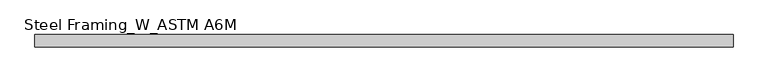
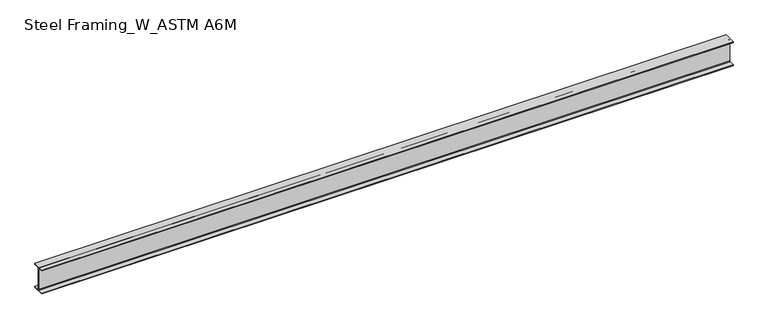
"""IFC4 building model written with IfcOpenShell, lengths in millimetres: beam geometry, Steel Framing_W_ASTM A6M : H_SB_AR_S02_W360x51_B4."""

from ifc_helpers import new_model, si_unit, point, frame, frame_2d, origin, place, context, project, spatial, polyline, circle_curve, trimmed, segment, composite_curve, outline, extrude, source, transform, mapped, element, save


def steel_framing_w_astm_a6m_8e55c2dc(model_context):
    return source(origin(), model_context, "Body", "SweptSolid", [
        extrude(outline(composite_curve([segment(polyline([(85.5, -166.4), (85.5, -178.0), (-85.5, -178.0), (-85.5, -166.4), (-13.72, -166.4)]), True, "CONTINUOUS"), segment(trimmed(circle_curve(frame_2d((-13.72, -156.3)), 10.1), [point((-13.72, -166.4))], [point((-3.62, -156.3))], True, "CARTESIAN"), True, "CONTINUOUS"), segment(polyline([(-3.62, -156.3), (-3.62, 156.3)]), True, "CONTINUOUS"), segment(trimmed(circle_curve(frame_2d((-13.72, 156.3)), 10.1), [point((-3.62, 156.3))], [point((-13.72, 166.4))], True, "CARTESIAN"), True, "CONTINUOUS"), segment(polyline([(-13.72, 166.4), (-85.5, 166.4), (-85.5, 178.0), (85.5, 178.0), (85.5, 166.4), (13.72, 166.4)]), True, "CONTINUOUS"), segment(trimmed(circle_curve(frame_2d((13.72, 156.3)), 10.1), [point((13.72, 166.4))], [point((3.62, 156.3))], True, "CARTESIAN"), True, "CONTINUOUS"), segment(polyline([(3.62, 156.3), (3.62, -156.3)]), True, "CONTINUOUS"), segment(trimmed(circle_curve(frame_2d((13.72, -156.3)), 10.1), [point((3.62, -156.3))], [point((13.72, -166.4))], True, "CARTESIAN"), True, "CONTINUOUS"), segment(polyline([(13.72, -166.4), (85.5, -166.4)]), True, "CONTINUOUS")], self_intersect=False)), frame((-4901.8, 0.0, 0.0), z_axis=(1.0, 0.0, 0.0), x_axis=(0.0, 1.0, 0.0)), (0.0, 0.0, 1.0), 9803.6),
    ])


if __name__ == "__main__":
    model = new_model("IFC4")
    model_context = context("Model", 3, world=origin())
    ifc_project = project(units=[si_unit("LENGTHUNIT", "METRE", prefix="MILLI")], contexts=[model_context])
    site = spatial("IfcSite", under=ifc_project)
    building = spatial("IfcBuilding", under=site)
    placement = place(None, origin())
    steel_framing_w_astm_a6m_shape = steel_framing_w_astm_a6m_8e55c2dc(model_context)
    element("IfcBeam", 1, ObjectType="Steel Framing_W_ASTM A6M : H_SB_AR_S02_W360x51_B4", at=placement, inside=building, context=model_context, shape_type="MappedRepresentation", body=[
        mapped(steel_framing_w_astm_a6m_shape, transform((0.0, 0.0, 0.0), x_axis=(1.0, 0.0, 0.0), y_axis=(0.0, 1.0, 0.0), z_axis=(0.0, 0.0, 1.0))),
    ])
    save(model, "model.ifc")

# Revit data of these elements
# Type "Steel Framing_W_ASTM A6M : H_SB_AR_S02_W360x51_B4"
#   Type Mark = "B4"
#   Section Name Key = "W14x34"
#   Width = 17.1 cm
#   Web Thickness = 0.724 cm
#   Web Fillet = 1.01 cm
#   Warping Constant = 287000.0 cm⁶
#   Torsional Moment of Inertia = 23.70 cm⁴
#   Section Area = 64.5 cm²
#   Plastic Modulus weak axis = 174.0 cm³
#   Plastic Modulus strong axis = 895.0 cm³
#   Perimeter = 1.36 m²/m
#   Nominal Weight = 51.00 kgf/m
#   Moment of Inertia weak axis = 970.00 cm⁴
#   Moment of Inertia strong axis = 14200.00 cm⁴
#   Height = 35.6 cm
#   Flange Thickness = 1.16 cm
#   Elastic Modulus weak axis = 113.0 cm³
#   Elastic Modulus strong axis = 796.0 cm³
#   Centroid Vertical = 17.8 cm
#   Centroid Horizontal = 8.55 cm
#   Length [instance default] = 1500 mm
#   Structural Material [instance default] = Steel, 45-345
#   Bolt Spacing = 0
#   Assembly Code = ""
# Element 1 (IfcBeam, "Steel Framing_W_ASTM A6M : H_SB_AR_S02_W360x51_B4")
#   Materials on its faces: "Steel, 45-345"
# Materials
#   "Steel, 45-345": class "Metal", colour RGB 189 187 185, transparency 0, Description = "Steel 345 MPa", Cost = 0
